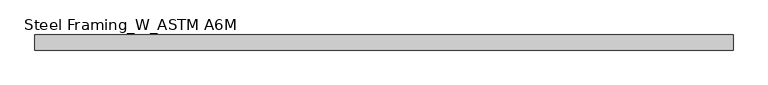
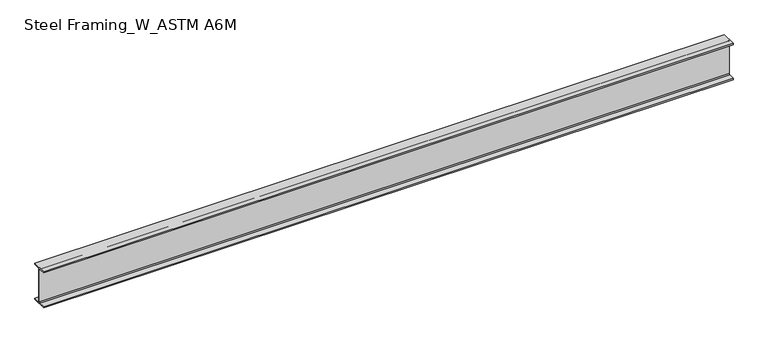
"""IFC4 building model written with IfcOpenShell, lengths in millimetres: beam geometry, Steel Framing_W_ASTM A6M : H_SB_AR_S02_W530x101_RB1."""

from ifc_helpers import new_model, si_unit, point, frame, frame_2d, origin, place, context, project, spatial, polyline, circle_curve, trimmed, segment, composite_curve, outline, extrude, source, transform, mapped, element, save


def steel_framing_w_astm_a6m_b326352c(model_context):
    return source(origin(), model_context, "Body", "SweptSolid", [
        extrude(outline(composite_curve([segment(polyline([(105.0, -250.6), (105.0, -268.0), (-105.0, -268.0), (-105.0, -250.6), (-18.25, -250.6)]), True, "CONTINUOUS"), segment(trimmed(circle_curve(frame_2d((-18.25, -237.8)), 12.8), [point((-18.25, -250.6))], [point((-5.45, -237.8))], True, "CARTESIAN"), True, "CONTINUOUS"), segment(polyline([(-5.45, -237.8), (-5.45, 237.8)]), True, "CONTINUOUS"), segment(trimmed(circle_curve(frame_2d((-18.25, 237.8)), 12.8), [point((-5.45, 237.8))], [point((-18.25, 250.6))], True, "CARTESIAN"), True, "CONTINUOUS"), segment(polyline([(-18.25, 250.6), (-105.0, 250.6), (-105.0, 268.0), (105.0, 268.0), (105.0, 250.6), (18.25, 250.6)]), True, "CONTINUOUS"), segment(trimmed(circle_curve(frame_2d((18.25, 237.8)), 12.8), [point((18.25, 250.6))], [point((5.45, 237.8))], True, "CARTESIAN"), True, "CONTINUOUS"), segment(polyline([(5.45, 237.8), (5.45, -237.8)]), True, "CONTINUOUS"), segment(trimmed(circle_curve(frame_2d((18.25, -237.8)), 12.8), [point((5.45, -237.8))], [point((18.25, -250.6))], True, "CARTESIAN"), True, "CONTINUOUS"), segment(polyline([(18.25, -250.6), (105.0, -250.6)]), True, "CONTINUOUS")], self_intersect=False)), frame((-4846.3, 0.0, 0.0), z_axis=(1.0, 0.0, 0.0), x_axis=(0.0, 1.0, 0.0)), (0.0, 0.0, 1.0), 9692.6),
    ])


if __name__ == "__main__":
    model = new_model("IFC4")
    model_context = context("Model", 3, world=origin())
    ifc_project = project(units=[si_unit("LENGTHUNIT", "METRE", prefix="MILLI")], contexts=[model_context])
    site = spatial("IfcSite", under=ifc_project)
    building = spatial("IfcBuilding", under=site)
    placement = place(None, origin())
    steel_framing_w_astm_a6m_shape = steel_framing_w_astm_a6m_b326352c(model_context)
    element("IfcBeam", 1, ObjectType="Steel Framing_W_ASTM A6M : H_SB_AR_S02_W530x101_RB1", at=placement, inside=building, context=model_context, shape_type="MappedRepresentation", body=[
        mapped(steel_framing_w_astm_a6m_shape, transform((0.0, 0.0, 0.0), x_axis=(1.0, 0.0, 0.0), y_axis=(0.0, 1.0, 0.0), z_axis=(0.0, 0.0, 1.0))),
    ])
    save(model, "model.ifc")

# Revit data of these elements
# Type "Steel Framing_W_ASTM A6M : H_SB_AR_S02_W530x101_RB1"
#   Type Mark = "RB1"
#   Section Name Key = "W21x68"
#   Width = 21.0 cm
#   Web Thickness = 1.09 cm
#   Web Fillet = 1.28 cm
#   Warping Constant = 1820000.0 cm⁶
#   Torsional Moment of Inertia = 102.00 cm⁴
#   Section Area = 129.0 cm²
#   Plastic Modulus weak axis = 400.0 cm³
#   Plastic Modulus strong axis = 2620.0 cm³
#   Perimeter = 1.87 m²/m
#   Nominal Weight = 101.00 kgf/m
#   Moment of Inertia weak axis = 2690.00 cm⁴
#   Moment of Inertia strong axis = 61600.00 cm⁴
#   Height = 53.6 cm
#   Flange Thickness = 1.74 cm
#   Elastic Modulus weak axis = 257.0 cm³
#   Elastic Modulus strong axis = 2290.0 cm³
#   Centroid Vertical = 26.8 cm
#   Centroid Horizontal = 10.5 cm
#   Length [instance default] = 1500 mm
#   Structural Material [instance default] = Steel, 45-345
#   Bolt Spacing = 0
#   Assembly Code = ""
# Element 1 (IfcBeam, "Steel Framing_W_ASTM A6M : H_SB_AR_S02_W530x101_RB1")
#   Materials on its faces: "Steel, 45-345"
# Materials
#   "Steel, 45-345": class "Metal", colour RGB 189 187 185, transparency 0, Description = "Steel 345 MPa", Cost = 0
